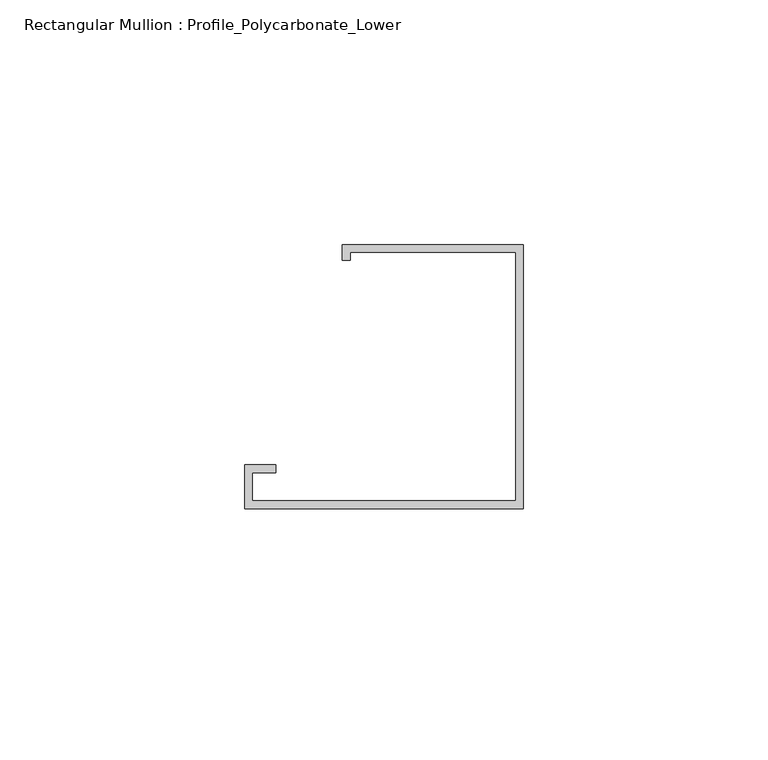
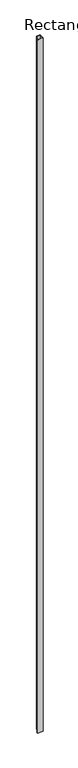
"""IFC4 building model written with IfcOpenShell, lengths in millimetres: member geometry, Rectangular Mullion : Profile_Polycarbonate_Lower."""

from ifc_helpers import new_model, si_unit, frame, origin, place, context, project, spatial, polyline, outline, extrude, source, transform, mapped, element, save


def rectangular_mullion_profile_polycarbonate_lower_8ce0784b(model_context):
    return source(origin(), model_context, "Body", "SweptSolid", [
        extrude(outline(polyline([(0.0, -28.984575), (-56.9976, -28.984575), (-56.9976, -19.992975), (-50.6476, -19.992975), (-50.6476, -21.580475), (-55.4101, -21.580475), (-55.4101, -27.397075), (-1.5875, -27.397075), (-1.5875, 23.428325), (-35.3949, 23.428325), (-35.3949, 21.840825), (-36.9824, 21.840825), (-36.9824, 25.015825), (0.0, 25.015825), (0.0, -28.984575)])), frame((0.0, 0.0, -7581.8043531), z_axis=(0.0, 0.0, 1.0), x_axis=(1.0, 0.0, 0.0)), (0.0, 0.0, 1.0), 7581.8043531),
    ])


if __name__ == "__main__":
    model = new_model("IFC4")
    model_context = context("Model", 3, world=origin())
    ifc_project = project(units=[si_unit("LENGTHUNIT", "METRE", prefix="MILLI")], contexts=[model_context])
    site = spatial("IfcSite", under=ifc_project)
    building = spatial("IfcBuilding", under=site)
    placement = place(None, origin())
    rectangular_mullion_profile_polycarbonate_lower_shape = rectangular_mullion_profile_polycarbonate_lower_8ce0784b(model_context)
    element("IfcMember", 1, ObjectType="Rectangular Mullion : Profile_Polycarbonate_Lower", at=placement, inside=building, context=model_context, shape_type="MappedRepresentation", body=[
        mapped(rectangular_mullion_profile_polycarbonate_lower_shape, transform((0.0, 0.0, 0.0), x_axis=(1.0, 0.0, 0.0), y_axis=(0.0, 1.0, 0.0), z_axis=(0.0, 0.0, 1.0))),
    ])
    save(model, "model.ifc")

# Revit data of these elements
# Type "Rectangular Mullion : Profile_Polycarbonate_Lower"
#   built-in parameter 1007322 = 0.177167 (stored number, unit not read)
#   built-in parameter 1007321 = 0 (stored number, unit not read)
#   built-in parameter 1007320 = 0.00520833 (stored number, unit not read)
